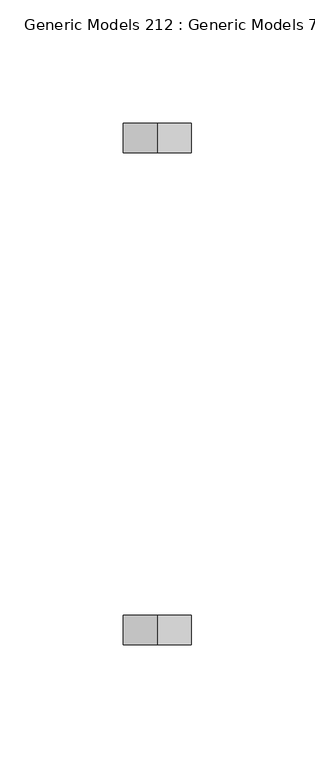
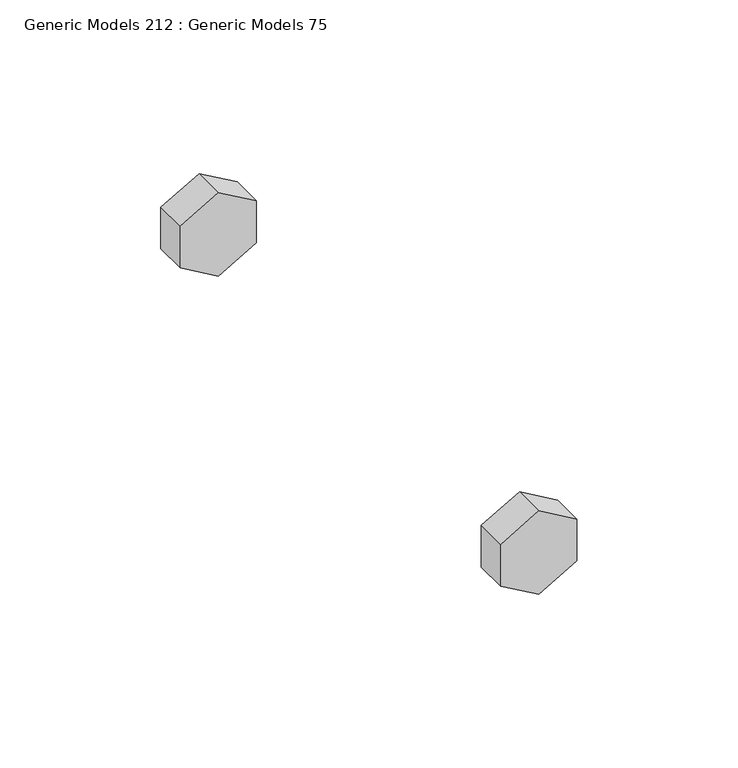
"""IFC4 building model written with IfcOpenShell, lengths in millimetres: proxy geometry, Generic Models 212 : Generic Models 75."""

from ifc_helpers import new_model, si_unit, frame, origin, place, context, project, spatial, polyline, outline, extrude, source, transform, mapped, element, save


def generic_models_212_generic_models_75_8fa15b82(model_context):
    return source(origin(), model_context, "Body", "SweptSolid", [
        extrude(outline(polyline([(268841.3462802, 31974.4067029), (268825.5097067, 31974.4067029), (268817.59142, 31988.1215778), (268825.5097067, 32001.8364528), (268841.3462802, 32001.8364528), (268849.264567, 31988.1215778), (268841.3462802, 31974.4067029)])), frame((0.0, 36501.0832942, 0.0), z_axis=(0.0, 1.0, 0.0), x_axis=(0.0, 0.0, 1.0)), (0.0, 0.0, 1.0), 11.90625),
        extrude(outline(polyline([(268841.3462802, 31974.4067029), (268825.5097067, 31974.4067029), (268817.59142, 31988.1215778), (268825.5097067, 32001.8364528), (268841.3462802, 32001.8364528), (268849.264567, 31988.1215778), (268841.3462802, 31974.4067029)])), frame((0.0, 36301.8520442, 0.0), z_axis=(0.0, 1.0, 0.0), x_axis=(0.0, 0.0, 1.0)), (0.0, 0.0, 1.0), 11.90625),
    ])


if __name__ == "__main__":
    model = new_model("IFC4")
    model_context = context("Model", 3, world=origin())
    ifc_project = project(units=[si_unit("LENGTHUNIT", "METRE", prefix="MILLI")], contexts=[model_context])
    site = spatial("IfcSite", under=ifc_project)
    building = spatial("IfcBuilding", under=site)
    placement = place(None, origin())
    generic_models_212_generic_models_75_shape = generic_models_212_generic_models_75_8fa15b82(model_context)
    element("IfcBuildingElementProxy", 1, Name="Generic Models 212 : Generic Models 75", ObjectType="Generic Models 212 : Generic Models 75", at=placement, inside=building, context=model_context, shape_type="MappedRepresentation", body=[
        mapped(generic_models_212_generic_models_75_shape, transform((0.0, 0.0, 0.0), x_axis=(1.0, 0.0, 0.0), y_axis=(0.0, 1.0, 0.0), z_axis=(0.0, 0.0, 1.0))),
    ])
    save(model, "model.ifc")

# Revit data of these elements
# Element 1 (IfcBuildingElementProxy, "Generic Models 212 : Generic Models 75")
#   Materials on its faces: "3/4\" GALV. THRU BOLTS"
# Materials
#   "3/4\" GALV. THRU BOLTS": class "Generic", colour RGB 105 69 171, transparency 0, Cost = 0
